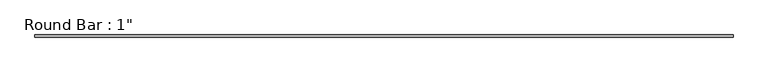
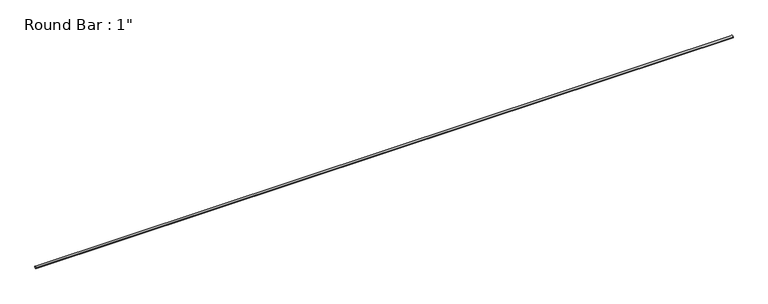
"""IFC4 building model written with IfcOpenShell, lengths in millimetres: member geometry."""

from ifc_helpers import new_model, si_unit, point, frame, origin, origin_2d, place, context, project, spatial, circle_curve, trimmed, segment, composite_curve, outline, extrude, source, transform, mapped, element, save


def member_91e7c94a(model_context):
    return source(origin(), model_context, "Body", "SweptSolid", [
        extrude(outline(composite_curve([segment(trimmed(circle_curve(origin_2d(), 12.7), [point((12.7, 0.0))], [point((-12.7, 0.0))], False, "CARTESIAN"), True, "CONTINUOUS"), segment(trimmed(circle_curve(origin_2d(), 12.7), [point((-12.7, 0.0))], [point((12.7, 0.0))], False, "CARTESIAN"), True, "CONTINUOUS")], self_intersect=False)), frame((-4095.75, 0.0, 0.0), z_axis=(1.0, 0.0, 0.0), x_axis=(0.0, 1.0, 0.0)), (0.0, 0.0, 1.0), 8191.5),
    ])


if __name__ == "__main__":
    model = new_model("IFC4")
    model_context = context("Model", 3, world=origin())
    ifc_project = project(units=[si_unit("LENGTHUNIT", "METRE", prefix="MILLI")], contexts=[model_context])
    site = spatial("IfcSite", under=ifc_project)
    building = spatial("IfcBuilding", under=site)
    placement = place(None, origin())
    member_shape = member_91e7c94a(model_context)
    element("IfcMember", 1, ObjectType="Round Bar : 1\"", at=placement, inside=building, context=model_context, shape_type="MappedRepresentation", body=[
        mapped(member_shape, transform((0.0, 0.0, 0.0), x_axis=(1.0, 0.0, 0.0), y_axis=(0.0, 1.0, 0.0), z_axis=(0.0, 0.0, 1.0))),
    ])
    save(model, "model.ifc")

# Revit data of these elements
# Type "Round Bar : 1\""
#   Assembly Code = "B10"
#   W = 0
#   Start Extension Calculation [instance default] = 10' - 0"
#   Start Extension [instance default] = -0' - 0 1/2"
#   End Extension Calculation [instance default] = 10' - 0"
#   End Extension [instance default] = -0' - 0 1/2"
#   Length [instance default] = 5' - 0"
#   d = 0' - 1"
#   A = 0 SF
#   Structural Material [instance default] = Metal - Steel - ASTM A36
# Element 1 (IfcMember, "Round Bar : 1\"")
#   Materials on its faces: "Metal - Steel - ASTM A36"
# Materials
#   "Metal - Steel - ASTM A36": class "Metal", colour RGB 199 199 199, transparency 0
